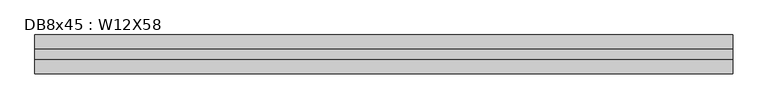
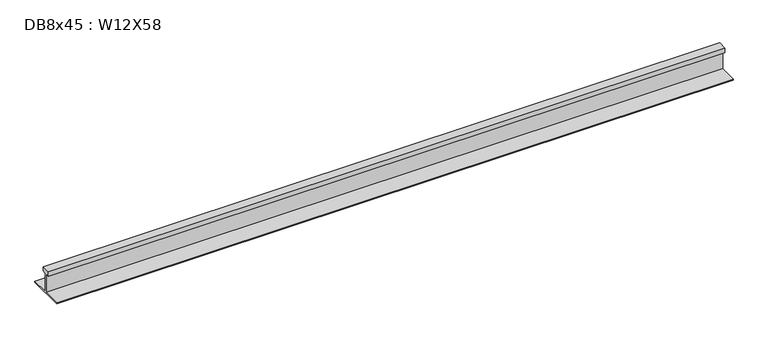
"""IFC4 building model written with IfcOpenShell, lengths in millimetres: beam geometry, DB8x45 : W12X58."""

from ifc_helpers import new_model, si_unit, frame, origin, place, context, project, spatial, polyline, outline, extrude, source, transform, mapped, element, save


def db8x45_w12x58_8a698736(model_context):
    return source(origin(), model_context, "Body", "SweptSolid", [
        extrude(outline(polyline([(38.1, 144.3355), (38.1, 106.2355), (4.7625, 106.2355), (4.7625, -49.53), (152.4, -49.53), (152.4, -59.182), (-152.4, -59.182), (-152.4, -49.53), (-4.7625, -49.53), (-4.7625, 106.2355), (-38.1, 106.2355), (-38.1, 144.3355), (38.1, 144.3355)])), frame((-2743.073, 0.0, 0.0), z_axis=(1.0, 0.0, 0.0), x_axis=(0.0, 1.0, 0.0)), (0.0, 0.0, 1.0), 5486.146),
    ])


if __name__ == "__main__":
    model = new_model("IFC4")
    model_context = context("Model", 3, world=origin())
    ifc_project = project(units=[si_unit("LENGTHUNIT", "METRE", prefix="MILLI")], contexts=[model_context])
    site = spatial("IfcSite", under=ifc_project)
    building = spatial("IfcBuilding", under=site)
    placement = place(None, origin())
    db8x45_w12x58_shape = db8x45_w12x58_8a698736(model_context)
    element("IfcBeam", 1, ObjectType="DB8x45 : W12X58", at=placement, inside=building, context=model_context, shape_type="MappedRepresentation", body=[
        mapped(db8x45_w12x58_shape, transform((0.0, 0.0, 0.0), x_axis=(1.0, 0.0, 0.0), y_axis=(0.0, 1.0, 0.0), z_axis=(0.0, 0.0, 1.0))),
    ])
    save(model, "model.ifc")

# Revit data of these elements
# Type "DB8x45 : W12X58"
#   Assembly Code = "B10"
#   W = 58
#   Length [instance default] = 5' - 0"
#   bf = 0' - 10"
#   d = 1' - 0.1"
#   k = 0' - 1 3/8"
#   k2 = 0' - 0.8"
#   tf = 0' - 0.575"
#   tw = 0' - 0.345"
#   A = 0.108333 SF
#   Structural Material [instance default] = Steel ASTM A992
# Element 1 (IfcBeam, "DB8x45 : W12X58")
#   Materials on its faces: "Steel ASTM A992"
# Materials
#   "Steel ASTM A992": class "Metal", colour RGB 199 199 199, transparency 0, Description = "Structural steel 50ksi", Cost = 0
